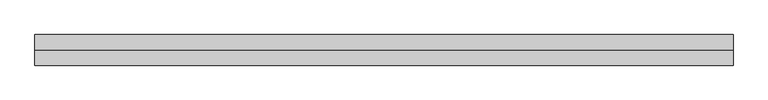
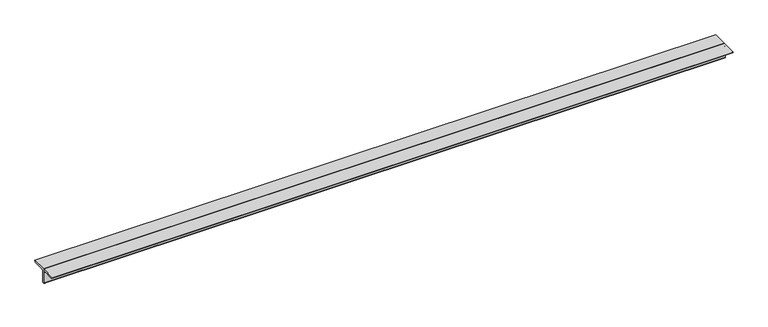
"""IFC4 building model written with IfcOpenShell, lengths in millimetres: member geometry, 0123_Steel Framing_2Ls-KSD3502 : H_SB_AR_S03_2Ls-130x130x12_HBR1."""

from ifc_helpers import new_model, si_unit, point, frame, frame_2d, origin, place, context, project, spatial, polyline, circle_curve, trimmed, segment, composite_curve, outline, extrude, source, transform, mapped, element, save


def member_fd7f8bdb(model_context):
    return source(origin(), model_context, "Body", "SweptSolid", [
        extrude(outline(composite_curve([segment(polyline([(0.0, 36.4), (130.0, 36.4)]), True, "CONTINUOUS"), segment(trimmed(circle_curve(frame_2d((118.0, 36.4)), 12.0), [point((130.0, 36.4))], [point((118.0, 24.4))], False, "CARTESIAN"), True, "CONTINUOUS"), segment(polyline([(118.0, 24.4), (24.0, 24.4)]), True, "CONTINUOUS"), segment(trimmed(circle_curve(frame_2d((24.0, 12.4)), 12.0), [point((24.0, 24.4))], [point((12.0, 12.4))], True, "CARTESIAN"), True, "CONTINUOUS"), segment(polyline([(12.0, 12.4), (12.0, -81.6)]), True, "CONTINUOUS"), segment(trimmed(circle_curve(frame_2d((0.0, -81.6)), 12.0), [point((12.0, -81.6))], [point((0.0, -93.6))], False, "CARTESIAN"), True, "CONTINUOUS"), segment(polyline([(0.0, -93.6), (0.0, 36.4)]), True, "CONTINUOUS")], self_intersect=False)), frame((-2923.1123523, 0.0, 0.0), z_axis=(1.0, 0.0, 0.0), x_axis=(0.0, 1.0, 0.0)), (0.0, 0.0, 1.0), 5929.4021426),
        extrude(outline(composite_curve([segment(polyline([(0.0, 36.4), (0.0, -93.6)]), True, "CONTINUOUS"), segment(trimmed(circle_curve(frame_2d((0.0, -81.6)), 12.0), [point((0.0, -93.6))], [point((-12.0, -81.6))], False, "CARTESIAN"), True, "CONTINUOUS"), segment(polyline([(-12.0, -81.6), (-12.0, 12.4)]), True, "CONTINUOUS"), segment(trimmed(circle_curve(frame_2d((-24.0, 12.4)), 12.0), [point((-12.0, 12.4))], [point((-24.0, 24.4))], True, "CARTESIAN"), True, "CONTINUOUS"), segment(polyline([(-24.0, 24.4), (-118.0, 24.4)]), True, "CONTINUOUS"), segment(trimmed(circle_curve(frame_2d((-118.0, 36.4)), 12.0), [point((-118.0, 24.4))], [point((-130.0, 36.4))], False, "CARTESIAN"), True, "CONTINUOUS"), segment(polyline([(-130.0, 36.4), (0.0, 36.4)]), True, "CONTINUOUS")], self_intersect=False)), frame((-2923.1123523, 0.0, 0.0), z_axis=(1.0, 0.0, 0.0), x_axis=(0.0, 1.0, 0.0)), (0.0, 0.0, 1.0), 5929.4021426),
    ])


if __name__ == "__main__":
    model = new_model("IFC4")
    model_context = context("Model", 3, world=origin())
    ifc_project = project(units=[si_unit("LENGTHUNIT", "METRE", prefix="MILLI")], contexts=[model_context])
    site = spatial("IfcSite", under=ifc_project)
    building = spatial("IfcBuilding", under=site)
    placement = place(None, origin())
    member_shape = member_fd7f8bdb(model_context)
    element("IfcMember", 1, ObjectType="0123_Steel Framing_2Ls-KSD3502 : H_SB_AR_S03_2Ls-130x130x12_HBR1", at=placement, inside=building, context=model_context, shape_type="MappedRepresentation", body=[
        mapped(member_shape, transform((0.0, 0.0, 0.0), x_axis=(1.0, 0.0, 0.0), y_axis=(0.0, 1.0, 0.0), z_axis=(0.0, 0.0, 1.0))),
    ])
    save(model, "model.ifc")

# Revit data of these elements
# Type "0123_Steel Framing_2Ls-KSD3502 : H_SB_AR_S03_2Ls-130x130x12_HBR1"
#   Type Mark = "HBR1"
#   Assembly Code = "B10"
#   Legs = "SLBB"
#   W = 8.97
#   Perimeter = 1.04 m²/m
#   Nominal Weight = 46.80 kgf/m
#   Length [instance default] = 1000 mm
#   Space = 0 mm
#   b = 130 mm
#   d = 130 mm
#   t = 12 mm
#   y = 36.4 mm
#   A = 0.005952 m²
#   Structural Material [instance default] = Steel ASTM A36
# Element 1 (IfcMember, "0123_Steel Framing_2Ls-KSD3502 : H_SB_AR_S03_2Ls-130x130x12_HBR1")
#   Materials on its faces: "Steel ASTM A36"
# Materials
#   "Steel ASTM A36": class "Metal", colour RGB 199 199 199, transparency 0, Description = "Structural steel, ASTM A36 Grade B, mill finish", Cost = 0
